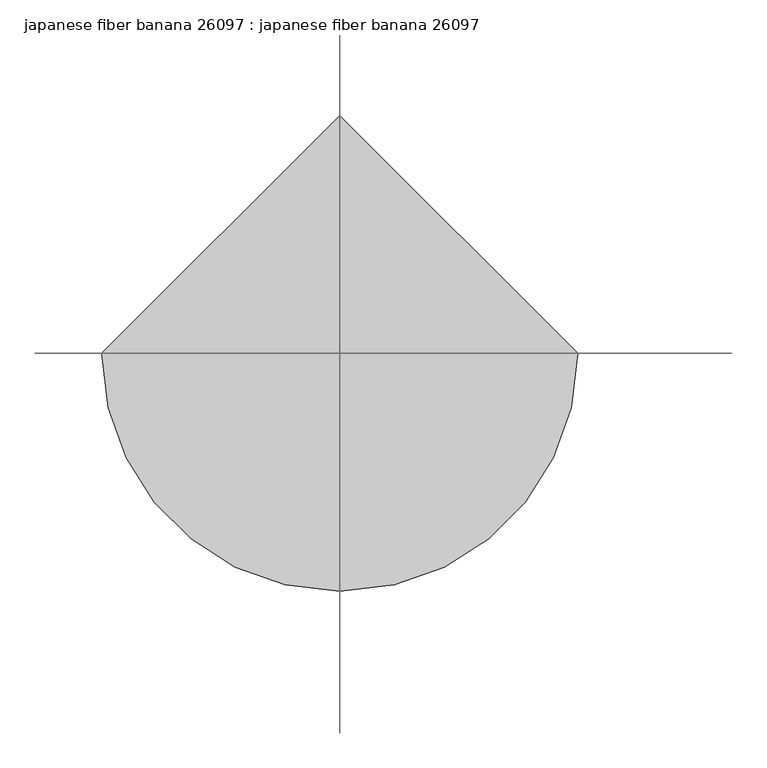
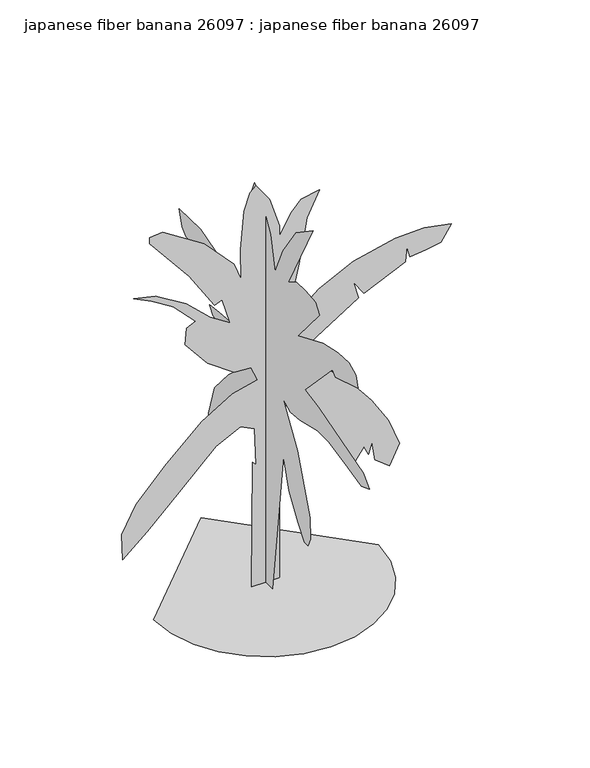
"""IFC4 building model written with IfcOpenShell, lengths in millimetres: proxy geometry, japanese fiber banana 26097 : japanese fiber banana 26097."""

from ifc_helpers import new_model, si_unit, origin, place, context, project, spatial, triangles, source, transform, mapped, element, save


def japanese_fiber_banana_26097_japanese_fiber_banana_26097_fc2fb2a9(model_context):
    return source(origin(), model_context, "Body", "Tessellation", [
        triangles([(-649.7467501, 0.0, 3.7e-06), (-632.5712723, -148.8792756, 3.7e-06), (-583.6506755, -285.6010629, 3.7e-06), (-506.9043426, -406.2488949, 3.7e-06), (-406.2488949, -506.9043426, 3.7e-06), (-285.6010629, -583.6506755, 3.7e-06), (-148.8792756, -632.5712723, 3.7e-06), (2.84e-05, -649.7467501, 3.7e-06), (148.8792756, -632.5712723, 3.7e-06), (285.6010629, -583.6506755, 3.7e-06), (406.2488949, -506.9043426, 3.7e-06), (506.9043426, -406.2488949, 3.7e-06), (583.6506755, -285.6010629, 3.7e-06), (632.5712723, -148.8790212, 3.7e-06), (649.7467501, 5.68e-05, 3.7e-06), (-8.52e-05, 649.7467501, 3.7e-06), (73.5169788, -2.4e-06, 1488.9400761), (86.1999983, -4e-06, 1501.9626823), (108.3956093, -6.3e-06, 1521.7797867), (138.5178168, -9.4e-06, 1547.2586094), (174.9816703, -1.3e-05, 1577.2688416), (216.2016834, -1.69e-05, 1610.6750874), (260.5921424, -2.12e-05, 1646.3444218), (306.5688237, -2.56e-05, 1683.149152), (505.0933339, -3.74e-05, 1782.4125698), (746.7776007, -4.41e-05, 1838.5162674), (915.0912369, -4.46e-05, 1842.831847), (1070.4584976, -4.1e-05, 1812.6209003), (1010.0392931, -3.02e-05, 1721.9908218), (923.7222507, -2.81e-05, 1704.7264687), (833.0921722, -2.71e-05, 1696.0954548), (815.8277464, -3.48e-05, 1760.832637), (807.1968052, -2.45e-05, 1674.5181381), (565.5150455, -1.17e-05, 1566.6237064), (505.0933339, -2.2e-05, 1652.9382053), (535.3041716, -9.6e-06, 1549.3592079), (250.4636001, 1.15e-05, 1372.4146305), (207.3058056, 2.02e-05, 1299.0465797), (457.6205775, 4.54e-05, 1087.573078), (608.672295, 6.81e-05, 897.679509), (707.9358582, 8.66e-05, 742.3123209), (772.6704969, 0.0001061, 578.3115755), (712.2512924, 0.00012, 461.7861663), (630.2496843, 0.0001123, 526.5233485), (612.9878019, 9.89e-05, 638.7333235), (591.4078691, 0.0001066, 573.9961049), (565.5150455, 0.0001, 630.1023823), (518.0422892, 0.0001082, 561.0496931), (237.5161527, 6.86e-05, 893.3640747), (99.411601, 4.9e-05, 1057.362204), (82.1486921, 4.08e-05, 1126.4148932), (77.8327038, 0.0001751, 0.0), (-81.8504909, 0.0001751, 0.0), (-77.5347659, 8.45e-05, 759.5742033), (-55.9558732, 8.71e-05, 737.996814), (-64.587582, 6.09e-05, 958.1012569), (-146.5871735, 5.57e-05, 1001.2585064), (-289.0071958, 6.39e-05, 932.2058172), (-500.4806794, 8.86e-05, 725.0478951), (-686.0587051, 0.0001097, 548.1032813), (-828.4769743, 0.0001241, 427.259858), (-832.7950247, 0.0001056, 582.6295896), (-750.7934166, 8.71e-05, 737.996814), (-573.8488029, 6.5e-05, 923.574876), (-371.0062786, 4.28e-05, 1109.1529381), (-194.0604295, 3e-05, 1217.044899), (-47.3244142, 2.59e-05, 1251.5712799), (-86.1662158, 1.56e-05, 1337.8882496), (-185.4289796, 1.46e-05, 1346.5192635), (-336.4799704, 1.7e-06, 1454.4136951), (-465.9543348, -1.73e-05, 1614.0963902), (-457.3233936, -2.87e-05, 1709.0419029), (-405.5326232, -3.18e-05, 1734.93727), (-535.0069877, -4.77e-05, 1868.7272141), (-660.1633381, -5.7e-05, 1946.4106991), (-763.7423355, -6.31e-05, 1998.1989624), (-638.583478, -5.95e-05, 1967.9881611), (-461.6388642, -4.67e-05, 1860.0962002), (-323.5335222, -3.12e-05, 1730.6218357), (-207.0078768, -2.25e-05, 1657.2536396), (-254.4808694, -4.1e-05, 1812.6209003), (-297.6381552, -3.9e-05, 1795.3590179), (-444.3744384, -6.62e-05, 2024.0943295), (-673.1097862, -9.91e-05, 2300.30247), (-673.1097862, -0.0001038, 2339.1442852), (-595.4261559, -0.0001043, 2343.4597195), (-358.0598668, -8.63e-05, 2192.4080383), (-185.4289796, -6.42e-05, 2006.8299763), (-142.2711851, -5.13e-05, 1898.9380154), (-146.5871735, -7.29e-05, 2080.198027), (-125.0082762, -0.0001002, 2308.9359547), (-90.4819498, -0.000112, 2408.1969017), (-55.9558732, -0.0001156, 2438.4078484), (21.7278389, -0.0001027, 2330.5132713), (77.8327038, -8.11e-05, 2149.2507889), (77.8327038, -7.39e-05, 2088.8315117), (146.8851113, -8.78e-05, 2205.3569572), (202.9900806, -9.5e-05, 2265.7760891), (310.8842943, -9.76e-05, 2287.3560219), (237.5161527, -8.01e-05, 2140.619775), (190.0426515, -4.87e-05, 1877.3580826), (142.5693864, -2.3e-05, 1661.5692192), (124.24932, -1.81e-05, 1620.2990639), (106.9864112, -1.34e-05, 1581.1042179), (91.8370452, -9.2e-06, 1546.0623161), (79.8586157, -5.8e-06, 1517.2485226), (72.1077807, -3.4e-06, 1496.740472), (69.6416885, -2.1e-06, 1486.6108578), (-6.07e-05, -228.3904198, 1972.5652073), (-6.46e-05, -305.2429235, 2016.4820034), (-6.49e-05, -396.7365758, 2020.139629), (-6.39e-05, -495.5454429, 2009.1616653), (-5.9e-05, -535.8019973, 1954.2670509), (-3.61e-05, -319.883527, 1698.0893738), (-4.56e-05, -568.7408298, 1804.2211224), (-4.86e-05, -718.786722, 1837.1573387), (-4.89e-05, -828.5760235, 1840.8175804), (-4.63e-05, -901.771483, 1811.5388443), (-4.01e-05, -920.0697121, 1742.0061699), (-3.38e-05, -696.8283966, 1672.4708794), (-3.65e-05, -667.5522039, 1701.7496155), (-1.06e-05, -393.0764068, 1412.635722), (-8.3e-06, -524.8241063, 1387.0172276), (3.5e-06, -974.9643265, 1255.2694553), (8.7e-06, -1037.1792789, 1196.7146719), (1.13e-05, -956.6660975, 1167.4360085), (8.7e-06, -821.2583015, 1196.7146719), (5.1e-06, -623.6354805, 1236.971299), (5.1e-06, -517.5038046, 1236.971299), (8.7e-06, -341.8393816, 1196.7146719), (9.7e-06, -246.688885, 1185.7342375), (6.4e-06, -169.8356182, 1222.3306229), (2.67e-05, -316.2233943, 995.4317545), (5.65e-05, -440.6507558, 662.4010649), (6.79e-05, -447.9710575, 534.3135707), (7.28e-05, -422.3525631, 479.4163765), (7.28e-05, -385.756105, 479.4163765), (6.53e-05, -323.5411526, 563.5896907), (5.32e-05, -232.0500619, 698.9975229), (3.75e-05, -177.1549025, 874.6619459), (5.84e-05, -147.8774926, 640.4427395), (0.0001157, -67.36457, 3.7e-06), (0.0001157, 82.6820898, 3.7e-06), (9.61e-05, 82.6820898, 219.5804016), (0.0001026, 64.3836201, 146.3870222), (7.84e-05, 35.1062147, 417.2039675), (4.99e-05, 35.1062147, 735.593981), (2.38e-05, 79.0221933, 1028.3680435), (2.8e-05, 174.1739435, 980.7936945), (4.14e-05, 331.5396469, 830.7452225), (5.19e-05, 430.3510211, 713.6355829), (5.84e-05, 444.9891174, 640.4427395), (5.58e-05, 470.6076118, 669.7214029), (6.33e-05, 466.9474792, 585.5480887), (6.01e-05, 529.1624316, 622.1445105), (6.5e-05, 551.1207933, 567.2498597), (5.45e-05, 573.0791914, 684.3594629), (3.75e-05, 514.5243716, 874.6619459), (2.28e-05, 375.4563704, 1039.3484779), (6.1e-06, 170.5143013, 1225.9908646), (1.8e-06, 272.9848271, 1273.567757), (-1.1e-06, 393.7545994, 1306.5039734), (2e-07, 459.6297209, 1291.8659134), (-1.1e-06, 529.1624316, 1306.5039734), (-5e-06, 565.7588533, 1350.4207695), (-6.4e-06, 466.9474792, 1365.0588295), (-7.7e-06, 254.6866163, 1379.6968895), (-1.32e-05, 331.5396469, 1441.911842), (-2.5e-05, 514.5243716, 1573.6594688), (-2.96e-05, 730.4453854, 1624.896603), (-2.96e-05, 799.9781324, 1624.896603), (-3.29e-05, 840.2346869, 1661.4929157), (-4.1e-05, 869.5133503, 1752.9841335), (-4.14e-05, 653.5923729, 1756.6442299), (-3.58e-05, 441.3289484, 1694.4292774), (-3.02e-05, 283.9652797, 1632.214325), (-1.62e-05, 108.2998484, 1474.8480583), (-5.35e-05, 152.215827, 1892.0520985), (-8.06e-05, 185.15287, 2195.804052), (-9.63e-05, 111.9594906, 2371.468475), (-9.01e-05, 46.0854001, 2301.9356552), (-7.67e-05, -45.4067079, 2151.889872), (-5.87e-05, -89.322691, 1950.6068092), (-7.44e-05, -169.8356182, 2126.2712322), (-9.14e-05, -301.5827909, 2316.5737152), (-0.0001016, -469.9294556, 2430.0231857)], [[15, 16, 1], [14, 15, 1], [14, 1, 2], [13, 14, 2], [13, 2, 3], [13, 3, 4], [12, 13, 4], [11, 12, 4], [11, 4, 5], [11, 5, 6], [11, 6, 7], [11, 7, 8], [11, 8, 9], [11, 9, 10], [75, 76, 77], [45, 46, 47], [53, 54, 55], [60, 61, 62], [98, 99, 100], [97, 98, 100], [27, 28, 29], [27, 29, 30], [47, 48, 49], [60, 62, 63], [59, 60, 63], [59, 63, 64], [58, 59, 64], [58, 64, 65], [74, 75, 77], [74, 77, 78], [73, 74, 78], [73, 78, 79], [42, 43, 44], [42, 44, 45], [41, 42, 45], [92, 93, 94], [91, 92, 94], [96, 97, 100], [96, 100, 101], [52, 53, 55], [51, 52, 55], [51, 55, 56], [57, 58, 65], [57, 65, 66], [57, 66, 67], [27, 30, 31], [27, 31, 32], [26, 27, 32], [84, 85, 86], [83, 84, 86], [83, 86, 87], [83, 87, 88], [82, 83, 88], [81, 82, 88], [81, 88, 89], [56, 57, 67], [51, 56, 67], [91, 94, 95], [90, 91, 95], [90, 95, 96], [89, 90, 96], [89, 96, 101], [89, 101, 102], [33, 34, 35], [32, 33, 35], [26, 32, 35], [25, 26, 35], [24, 25, 35], [81, 89, 102], [80, 81, 102], [80, 102, 103], [80, 103, 104], [80, 104, 105], [80, 105, 106], [80, 106, 107], [40, 41, 45], [40, 45, 47], [40, 47, 49], [39, 40, 49], [38, 39, 49], [38, 49, 50], [38, 50, 51], [38, 51, 67], [38, 67, 68], [35, 36, 37], [24, 35, 37], [23, 24, 37], [22, 23, 37], [21, 22, 37], [20, 21, 37], [19, 20, 37], [18, 19, 37], [17, 18, 37], [17, 37, 38], [17, 38, 68], [108, 17, 68], [80, 107, 108], [80, 108, 68], [80, 68, 69], [80, 69, 70], [80, 70, 71], [79, 80, 71], [73, 79, 71], [73, 71, 72], [143, 144, 145], [185, 186, 109], [184, 185, 109], [155, 156, 157], [183, 184, 109], [151, 152, 153], [153, 154, 155], [164, 165, 166], [163, 164, 166], [124, 125, 126], [179, 180, 181], [172, 173, 174], [171, 172, 174], [170, 171, 174], [169, 170, 174], [169, 174, 175], [142, 143, 145], [141, 142, 145], [141, 145, 146], [141, 146, 147], [140, 141, 147], [140, 147, 148], [162, 163, 166], [162, 166, 167], [161, 162, 167], [179, 181, 182], [178, 179, 182], [178, 182, 183], [153, 155, 157], [153, 157, 158], [151, 153, 158], [150, 151, 158], [150, 158, 159], [149, 150, 159], [149, 159, 160], [148, 149, 160], [124, 126, 127], [123, 124, 127], [123, 127, 128], [123, 128, 129], [118, 119, 120], [117, 118, 120], [116, 117, 120], [116, 120, 121], [115, 116, 121], [115, 121, 122], [114, 115, 122], [168, 169, 175], [168, 175, 176], [168, 176, 177], [167, 168, 177], [177, 178, 183], [122, 123, 129], [122, 129, 130], [112, 113, 114], [111, 112, 114], [110, 111, 114], [109, 110, 114], [183, 109, 114], [177, 183, 114], [177, 114, 122], [177, 122, 130], [177, 130, 131], [177, 131, 132], [167, 177, 132], [161, 167, 132], [160, 161, 132], [148, 160, 132], [140, 148, 132], [140, 132, 133], [140, 133, 134], [139, 140, 134], [138, 139, 134], [138, 134, 135], [137, 138, 135], [137, 135, 136]], closed=False),
    ])


if __name__ == "__main__":
    model = new_model("IFC4")
    model_context = context("Model", 3, world=origin())
    ifc_project = project(units=[si_unit("LENGTHUNIT", "METRE", prefix="MILLI")], contexts=[model_context])
    site = spatial("IfcSite", under=ifc_project)
    building = spatial("IfcBuilding", under=site)
    placement = place(None, origin())
    japanese_fiber_banana_26097_japanese_fiber_banana_26097_shape = japanese_fiber_banana_26097_japanese_fiber_banana_26097_fc2fb2a9(model_context)
    element("IfcBuildingElementProxy", 1, Name="japanese fiber banana 26097 : japanese fiber banana 26097", ObjectType="japanese fiber banana 26097 : japanese fiber banana 26097", at=placement, inside=building, context=model_context, shape_type="MappedRepresentation", body=[
        mapped(japanese_fiber_banana_26097_japanese_fiber_banana_26097_shape, transform((0.0, 0.0, 0.0), x_axis=(1.0, 0.0, 0.0), y_axis=(0.0, 1.0, 0.0), z_axis=(0.0, 0.0, 1.0))),
    ])
    save(model, "model.ifc")

# Revit data of these elements
# Type "japanese fiber banana 26097 : japanese fiber banana 26097"
#   built-in parameter 1005195 = "RPC-16-FVGT-NR7X-7G1M-A000-ST1L-LVER-AU"
#   Height = 0
